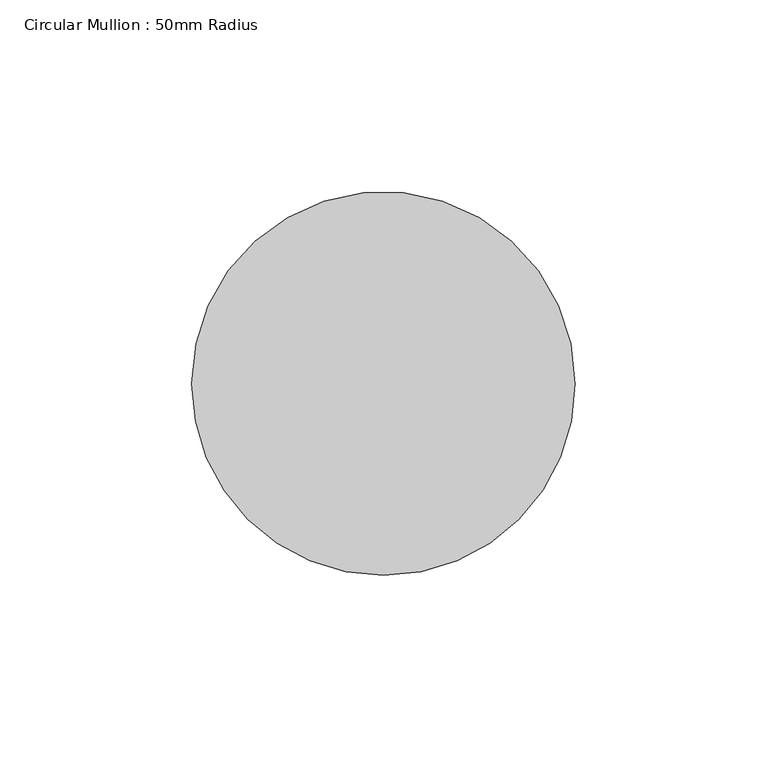
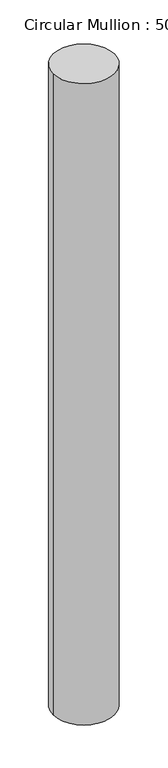
"""IFC4 building model written with IfcOpenShell, lengths in millimetres: member geometry, Circular Mullion : 50mm Radius."""

from ifc_helpers import new_model, si_unit, frame, origin, place, context, project, spatial, ellipse_curve, source, transform, mapped, element, save
from ifc_brep_helpers import plane_surface, cylinder_surface, advanced_brep


def circular_mullion_50mm_radius_0eb11e00(model_context):
    return source(origin(), model_context, "Body", "AdvancedBrep", [
        advanced_brep(
        [(-100.0, 0.0, 1.0623221), (0.0, 0.0, 0.0), (0.0, 0.0, -1099.8387195), (-100.0, 0.0, -1100.8628365)],
        [
            (0, 1, ellipse_curve(frame((-50.0, 0.0, 0.5311611), z_axis=(-0.010621476463060922, -0.014683392467561661, -0.9998357776272002), x_axis=(-0.5860035352354919, -0.8101058195784632, 0.018122300533097546)), 50.0082125, 50.0)),
            (1, 2),
            (2, 3, ellipse_curve(frame((-50.0, 0.0, -1100.350778), z_axis=(-0.010239607022274, -0.014155486682531419, 0.9998473746751602), x_axis=(0.5860103322627414, 0.8101152159576573, 0.017470757144149928)), 50.0076324, 50.0)),
            (3, 0),
            (1, 0, ellipse_curve(frame((-50.0, 0.0, 0.5311611), z_axis=(-0.010621476463060922, -0.014683392467561661, -0.9998357776272002), x_axis=(-0.5860035352354919, -0.8101058195784632, 0.018122300533097546)), 50.0082125, 50.0)),
            (3, 2, ellipse_curve(frame((-50.0, 0.0, -1100.350778), z_axis=(-0.010239607022274, -0.014155486682531419, 0.9998473746751602), x_axis=(0.5860103322627414, 0.8101152159576573, 0.017470757144149928)), 50.0076324, 50.0)),
        ],
        [
            cylinder_surface(frame((-50.0, 0.0, 0.0), z_axis=(0.0, 0.0, 1.0), x_axis=(1.0, 0.0, 0.0)), 50.0),
            plane_surface(frame((-246.9608103, 178.6432148, 0.0), z_axis=(0.010621476463060922, 0.014683392467561661, 0.9998357776272002), x_axis=(0.5860035352354906, 0.8101058195784642, -0.018122300533094677))),
            plane_surface(frame((-246.9608103, 178.6432148, -1099.8387195), z_axis=(0.010239607022274002, 0.014155486682531422, -0.9998473746751604), x_axis=(0.5860103322627414, 0.8101152159576573, 0.017470757144151694))),
        ],
        [
            (0, [[1, 2, 3, 4]]),
            (0, [[5, -4, 6, -2]]),
            (1, [[-1, -5]]),
            (2, [[-6, -3]]),
        ],
    ),
    ])


if __name__ == "__main__":
    model = new_model("IFC4")
    model_context = context("Model", 3, world=origin())
    ifc_project = project(units=[si_unit("LENGTHUNIT", "METRE", prefix="MILLI")], contexts=[model_context])
    site = spatial("IfcSite", under=ifc_project)
    building = spatial("IfcBuilding", under=site)
    placement = place(None, origin())
    circular_mullion_50mm_radius_shape = circular_mullion_50mm_radius_0eb11e00(model_context)
    element("IfcMember", 1, ObjectType="Circular Mullion : 50mm Radius", at=placement, inside=building, context=model_context, shape_type="MappedRepresentation", body=[
        mapped(circular_mullion_50mm_radius_shape, transform((0.0, 0.0, 0.0), x_axis=(1.0, 0.0, 0.0), y_axis=(0.0, 1.0, 0.0), z_axis=(0.0, 0.0, 1.0))),
    ])
    save(model, "model.ifc")

# Revit data of these elements
# Type "Circular Mullion : 50mm Radius"
#   built-in parameter 1007350 = 0.164042 (stored number, unit not read)
# Element 1 (IfcMember, "Circular Mullion : 50mm Radius")
#   Materials on its faces: "Aluminium"
# Materials
#   "Aluminium": class "Metal", colour RGB 247 247 247, transparency 0, Description = "Aluminium 6061", Cost = 0
